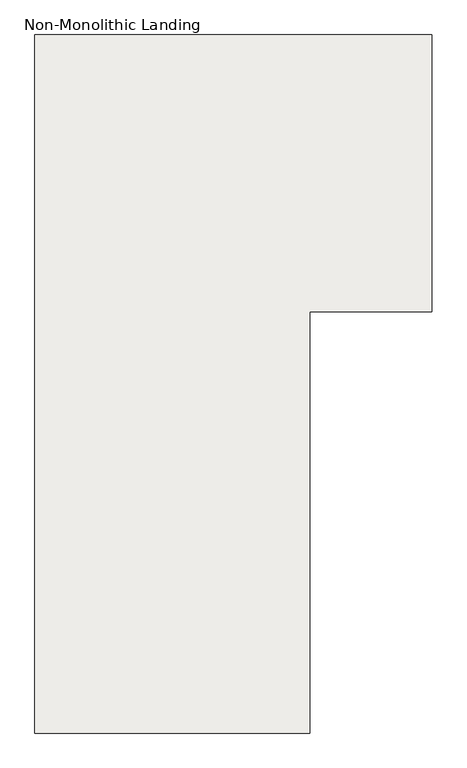
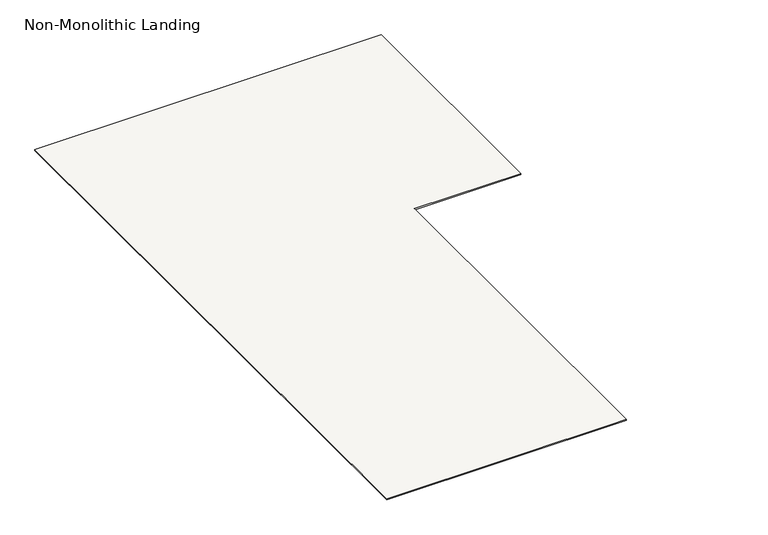
"""IFC4 building model written with IfcOpenShell, lengths in millimetres: slab geometry, Non-Monolithic Landing."""

from ifc_helpers import new_model, si_unit, origin, place, context, project, spatial, faceted_brep, source, transform, mapped, element, save


def non_monolithic_landing_addf079d(model_context):
    return source(origin(), model_context, "Body", "Brep", [
        faceted_brep([(14150.0, 13220.4345331, 20000.0), (12444.9411574, 13220.4345331, 20000.0), (12444.9411574, 10220.4345331, 20000.0), (13625.0, 10220.4345331, 20000.0), (13625.0, 12030.4345331, 20000.0), (14150.0, 12030.4345331, 20000.0), (12444.9411574, 10220.4345331, 19994.0), (12444.9411574, 13220.4345331, 19994.0), (14149.15, 13220.4345331, 19994.0), (14149.15, 12030.4345331, 19994.0), (13625.0, 12030.4345331, 19994.0), (13625.0, 10220.4345331, 19994.0)], [[[0, 1, 2, 3, 4, 5]], [[6, 7, 8, 9, 10, 11]], [[1, 0, 8, 7]], [[5, 4, 10, 9]], [[4, 3, 11, 10]], [[3, 2, 6, 11]], [[2, 1, 7, 6]], [[0, 5, 9, 8]]]),
    ])


if __name__ == "__main__":
    model = new_model("IFC4")
    model_context = context("Model", 3, world=origin())
    ifc_project = project(units=[si_unit("LENGTHUNIT", "METRE", prefix="MILLI")], contexts=[model_context])
    site = spatial("IfcSite", under=ifc_project)
    building = spatial("IfcBuilding", under=site)
    placement = place(None, origin())
    non_monolithic_landing_shape = non_monolithic_landing_addf079d(model_context)
    element("IfcSlab", 1, ObjectType="Non-Monolithic Landing", at=placement, inside=building, context=model_context, shape_type="MappedRepresentation", body=[
        mapped(non_monolithic_landing_shape, transform((0.0, 0.0, 0.0), x_axis=(1.0, 0.0, 0.0), y_axis=(0.0, 1.0, 0.0), z_axis=(0.0, 0.0, 1.0))),
    ])
    save(model, "model.ifc")

# Revit data of these elements
# Element 1 (IfcSlab, "Non-Monolithic Landing")
#   Materials on its faces: "Steel, Paint Finish, Dark Gray"
# Materials
#   "Steel, Paint Finish, Dark Gray": class "Metal", colour RGB 89 89 89, transparency 0, Description = "Steel, paint finish, dark gray, glossy", Cost = 0
